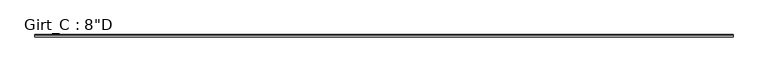
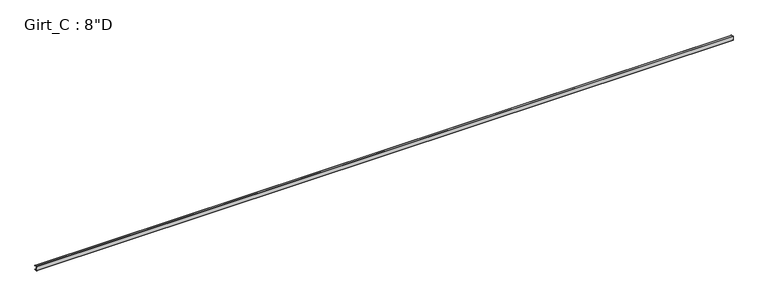
"""IFC4 building model written with IfcOpenShell, lengths in millimetres: beam geometry."""

from ifc_helpers import new_model, si_unit, point, frame, frame_2d, origin, place, context, project, spatial, polyline, circle_curve, trimmed, segment, composite_curve, outline, extrude, source, transform, mapped, element, save


def beam_b6572ddd(model_context):
    return source(origin(), model_context, "Body", "SweptSolid", [
        extrude(outline(composite_curve([segment(polyline([(87.5109375, 101.6), (99.7560415, 87.0068534), (97.6278742, 85.221109), (86.2154765, 98.821875), (3.3005807, 98.821875)]), True, "CONTINUOUS"), segment(trimmed(circle_curve(frame_2d((3.3741066, 96.8381931)), 1.9850441), [point((3.3005807, 98.821875))], [point((1.3890625, 96.8381931))], True, "CARTESIAN"), True, "CONTINUOUS"), segment(polyline([(1.3890625, 96.8381931), (1.3890625, -96.8389339)]), True, "CONTINUOUS"), segment(trimmed(circle_curve(frame_2d((3.3748024, -96.8389339)), 1.9857399), [point((1.3890625, -96.8389339))], [point((3.2694106, -98.821875))], True, "CARTESIAN"), True, "CONTINUOUS"), segment(polyline([(3.2694106, -98.821875), (86.2154765, -98.821875), (97.6510975, -85.1934327), (99.7792647, -86.979177), (87.5109375, -101.6), (3.3734375, -101.6)]), True, "CONTINUOUS"), segment(trimmed(circle_curve(frame_2d((3.3734375, -96.8375)), 4.7625), [point((3.3734375, -101.6))], [point((-1.3890625, -96.8375))], False, "CARTESIAN"), True, "CONTINUOUS"), segment(polyline([(-1.3890625, -96.8375), (-1.3890625, 96.8375)]), True, "CONTINUOUS"), segment(trimmed(circle_curve(frame_2d((3.3734375, 96.8375)), 4.7625), [point((-1.3890625, 96.8375))], [point((3.3734375, 101.6))], False, "CARTESIAN"), True, "CONTINUOUS"), segment(polyline([(3.3734375, 101.6), (87.5109375, 101.6)]), True, "CONTINUOUS")], self_intersect=False)), frame((-15570.2, 0.0, 0.0), z_axis=(1.0, 0.0, 0.0), x_axis=(0.0, 1.0, 0.0)), (0.0, 0.0, 1.0), 31140.4),
    ])


if __name__ == "__main__":
    model = new_model("IFC4")
    model_context = context("Model", 3, world=origin())
    ifc_project = project(units=[si_unit("LENGTHUNIT", "METRE", prefix="MILLI")], contexts=[model_context])
    site = spatial("IfcSite", under=ifc_project)
    building = spatial("IfcBuilding", under=site)
    placement = place(None, origin())
    beam_shape = beam_b6572ddd(model_context)
    element("IfcBeam", 1, ObjectType="Girt_C : 8\"D", at=placement, inside=building, context=model_context, shape_type="MappedRepresentation", body=[
        mapped(beam_shape, transform((0.0, 0.0, 0.0), x_axis=(1.0, 0.0, 0.0), y_axis=(0.0, 1.0, 0.0), z_axis=(0.0, 0.0, 1.0))),
    ])
    save(model, "model.ifc")

# Revit data of these elements
# Type "Girt_C : 8\"D"
#   half leg = 0' - 1 3/4"
#   Web_Thickness = 0' - 0 7/64"
#   Length [instance default] = 10' - 0"
#   Leg_1 = 0' - 3 1/2"
#   Height = 0' - 8"
#   Structural Material [instance default] = none
# Element 1 (IfcBeam, "Girt_C : 8\"D")
#   Structural Material = CEE' SECTION (8.0x3.5C - SEE STRUCT. DWGS)
#   Materials on its faces: "CEE' SECTION (8.0x3.5C - SEE STRUCT. DWGS)"
# Materials
#   "CEE' SECTION (8.0x3.5C - SEE STRUCT. DWGS)": class "Metal", colour RGB 137 146 153, transparency 0, Description = "Steel, mill finish", Cost = 0
